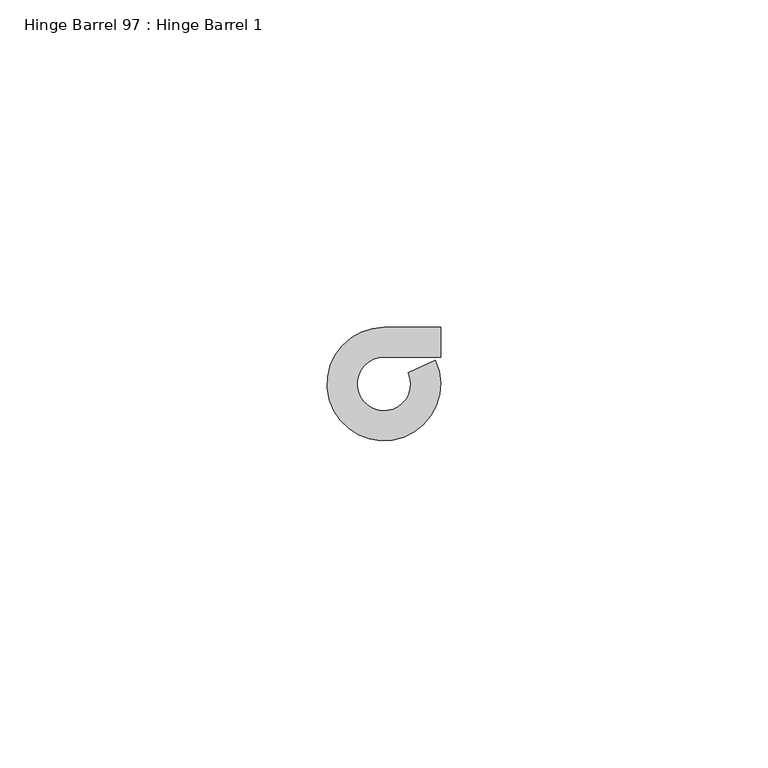
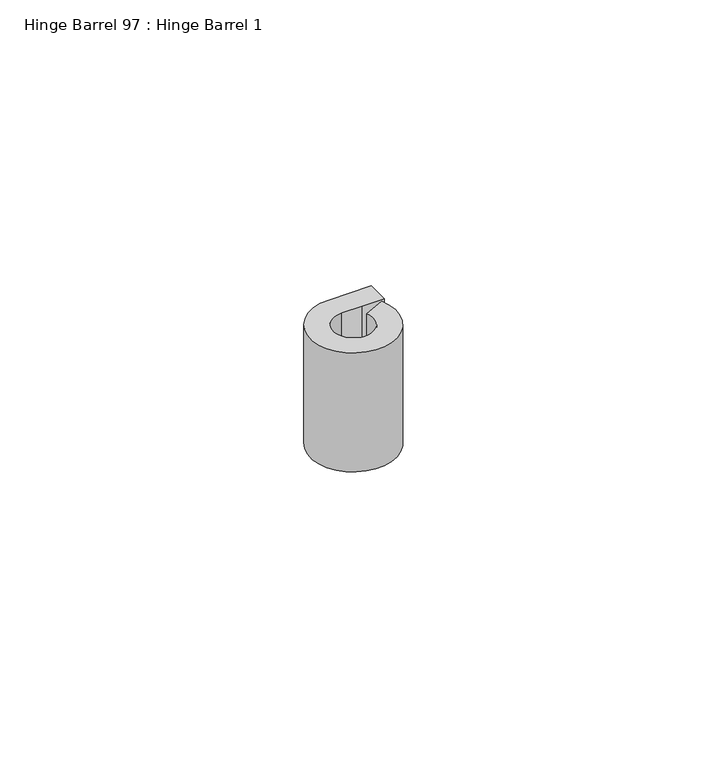
"""IFC4 building model written with IfcOpenShell, lengths in millimetres: proxy geometry, Hinge Barrel 97 : Hinge Barrel 1."""

from ifc_helpers import new_model, si_unit, point, frame, frame_2d, origin, place, context, project, spatial, polyline, circle_curve, trimmed, segment, composite_curve, outline, extrude, source, transform, mapped, element, save


def hinge_barrel_97_hinge_barrel_1_935fc850(model_context):
    return source(origin(), model_context, "Body", "SweptSolid", [
        extrude(outline(composite_curve([segment(polyline([(587323.2214739, -533980.5883841), (587319.1320739, -533980.5883841)]), True, "CONTINUOUS"), segment(trimmed(circle_curve(frame_2d((587319.1320739, -533984.6777841)), 4.0894), [point((587319.1320739, -533980.5883841))], [point((587322.8436736, -533982.9610371))], True, "CARTESIAN"), True, "CONTINUOUS"), segment(polyline([(587322.8436736, -533982.9610371), (587326.986084, -533981.0450249)]), True, "CONTINUOUS"), segment(trimmed(circle_curve(frame_2d((587319.1320739, -533984.6777841)), 8.6534625), [point((587326.986084, -533981.0450249))], [point((587319.1320739, -533976.0243216))], False, "CARTESIAN"), True, "CONTINUOUS"), segment(polyline([(587319.1320739, -533976.0243216), (587327.7934739, -533976.0243216), (587327.7934739, -533980.5883841), (587323.2214739, -533980.5883841)]), True, "CONTINUOUS")], self_intersect=False)), frame((0.0, 0.0, 1936.75), z_axis=(0.0, 0.0, 1.0), x_axis=(1.0, 0.0, 0.0)), (0.0, 0.0, 1.0), 25.4),
    ])


if __name__ == "__main__":
    model = new_model("IFC4")
    model_context = context("Model", 3, world=origin())
    ifc_project = project(units=[si_unit("LENGTHUNIT", "METRE", prefix="MILLI")], contexts=[model_context])
    site = spatial("IfcSite", under=ifc_project)
    building = spatial("IfcBuilding", under=site)
    placement = place(None, origin())
    hinge_barrel_97_hinge_barrel_1_shape = hinge_barrel_97_hinge_barrel_1_935fc850(model_context)
    element("IfcBuildingElementProxy", 1, Name="Hinge Barrel 97 : Hinge Barrel 1", ObjectType="Hinge Barrel 97 : Hinge Barrel 1", at=placement, inside=building, context=model_context, shape_type="MappedRepresentation", body=[
        mapped(hinge_barrel_97_hinge_barrel_1_shape, transform((0.0, 0.0, 0.0), x_axis=(1.0, 0.0, 0.0), y_axis=(0.0, 1.0, 0.0), z_axis=(0.0, 0.0, 1.0))),
    ])
    save(model, "model.ifc")

# Revit data of these elements
# Element 1 (IfcBuildingElementProxy, "Hinge Barrel 97 : Hinge Barrel 1")
#   Materials on its faces: "6\"X6\" WELD-ON STL BUTT HINGE"
# Materials
#   "6\"X6\" WELD-ON STL BUTT HINGE": class "Metal", colour RGB 189 187 185, transparency 0, Description = "Carbon steel", Cost = 0
